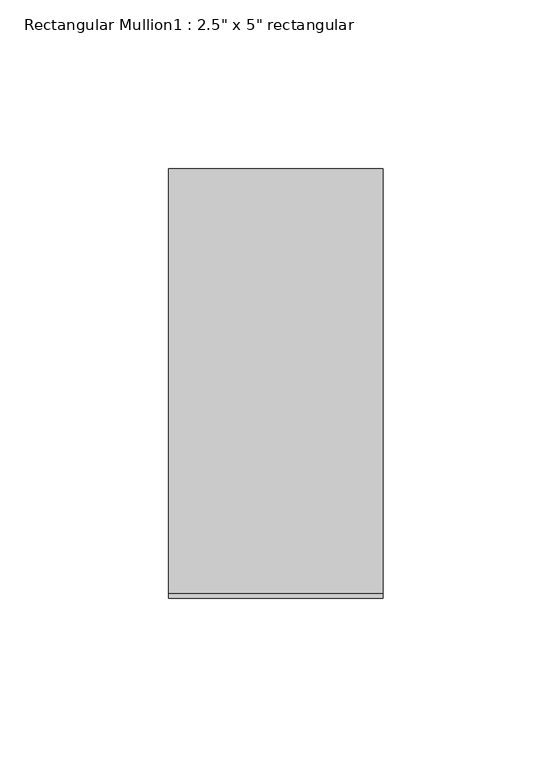
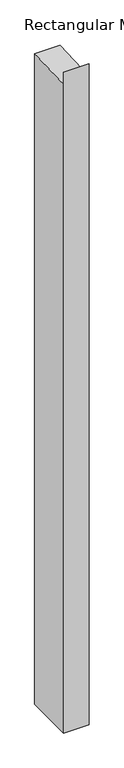
"""IFC4 building model written with IfcOpenShell, lengths in millimetres: member geometry."""

import ifcopenshell
import ifcopenshell.guid

model = None  # the IFC model being written
_history = None  # IfcOwnerHistory: only IFC2X3 demands one
_inside = {}  # id of a spatial element -> (the spatial element, [elements in it])
_under = {}  # id of a project, library or spatial element -> (it, [spatial elements below it])
_declared = {}  # id of a project -> (the project, [libraries it declares])
_typed = {}  # id of a type object -> (the type object, [elements of that type])
_made_of = {}  # id of a material, layer set ... -> (it, [elements and type objects made of it])


def new_model(schema):
    """Start an empty IFC model of exactly this schema.

    Asked for "IFC4X3", IfcOpenShell would pick the latest addendum, in which some entities
    have other attributes; the version numbers below select the first issue.
    IFC2X3 requires an IfcOwnerHistory on every rooted entity: one is made here for all.
    """
    global model, _history
    if schema == "IFC4X3":
        model = ifcopenshell.file(schema_version=(4, 3, 0, 0))
    else:
        model = ifcopenshell.file(schema=schema)
    _inside.clear()
    _under.clear()
    _declared.clear()
    _typed.clear()
    _made_of.clear()
    _history = None
    if model.schema == "IFC2X3":
        org = make("IfcOrganization", Name="unknown")
        user = make(
            "IfcPersonAndOrganization",
            ThePerson=make("IfcPerson", FamilyName="unknown"),
            TheOrganization=org,
        )
        app = make(
            "IfcApplication",
            ApplicationDeveloper=org,
            Version="unknown",
            ApplicationFullName="unknown",
            ApplicationIdentifier="unknown",
        )
        _history = make(
            "IfcOwnerHistory",
            OwningUser=user,
            OwningApplication=app,
            ChangeAction="ADDED",
            CreationDate=0,
        )
    return model


def make(cls, **values):
    """One entity of the class cls with the attributes given. An attribute that is None is left unset."""
    return model.create_entity(
        cls, **{name: value for name, value in values.items() if value is not None}
    )


def rooted(cls, **values):
    """An entity with a GlobalId (a new one), such as an element, a storey or a relation."""
    return make(cls, GlobalId=ifcopenshell.guid.new(), OwnerHistory=_history, **values)


def si_unit(unit_type, name, prefix=None):
    """IfcSIUnit, for example si_unit("LENGTHUNIT", "METRE", prefix="MILLI")."""
    return make("IfcSIUnit", UnitType=unit_type, Prefix=prefix, Name=name)


def assignment(units):
    """IfcUnitAssignment: the units of a project."""
    return None if units is None else make("IfcUnitAssignment", Units=units)


def point(xyz):
    """IfcCartesianPoint."""
    return None if xyz is None else make("IfcCartesianPoint", Coordinates=xyz)


def direction(xyz):
    """IfcDirection."""
    return None if xyz is None else make("IfcDirection", DirectionRatios=xyz)


def frame(location, z_axis=None, x_axis=None):
    """IfcAxis2Placement3D, a coordinate frame: its origin and axes. An axis left out is left unset."""
    return make(
        "IfcAxis2Placement3D",
        Location=point(location),
        Axis=direction(z_axis),
        RefDirection=direction(x_axis),
    )


def origin():
    """The frame at (0, 0, 0) with its axes left unset."""
    return frame((0.0, 0.0, 0.0))


def place(relative_to, where):
    """IfcLocalPlacement: puts the frame where relative to a parent placement (None: the world)."""
    return make(
        "IfcLocalPlacement", PlacementRelTo=relative_to, RelativePlacement=where
    )


def context(
    kind, dimensions, precision=None, world=None, true_north=None, identifier=None
):
    """IfcGeometricRepresentationContext, for example the 3D "Model" context."""
    return make(
        "IfcGeometricRepresentationContext",
        ContextIdentifier=identifier,
        ContextType=kind,
        CoordinateSpaceDimension=dimensions,
        Precision=precision,
        WorldCoordinateSystem=world,
        TrueNorth=true_north,
    )


def project(units=None, contexts=None):
    """IfcProject with its units and contexts."""
    return rooted(
        "IfcProject",
        Name="project",
        RepresentationContexts=contexts,
        UnitsInContext=assignment(units),
    )


def spatial(cls, under=None, at=None, **own):
    """A site, building, storey or space (cls), placed at a placement, below another one or the project."""
    s = rooted(cls, ObjectPlacement=at, **own)
    if under is not None:
        _under.setdefault(under.id(), (under, []))[1].append(s)
    return s


def polyline(points):
    """IfcPolyline through the points."""
    return make("IfcPolyline", Points=[point(p) for p in points])


def outline(outer, holes=None, kind="AREA"):
    """IfcArbitraryClosedProfileDef: a profile drawn as a closed curve; with holes, ...WithVoids."""
    if holes is None:
        return make("IfcArbitraryClosedProfileDef", ProfileType=kind, OuterCurve=outer)
    return make(
        "IfcArbitraryProfileDefWithVoids",
        ProfileType=kind,
        OuterCurve=outer,
        InnerCurves=holes,
    )


def extrude(swept, where, along, depth):
    """IfcExtrudedAreaSolid: the profile swept, set in the frame where, extruded along a direction by depth."""
    return make(
        "IfcExtrudedAreaSolid",
        SweptArea=swept,
        Position=where,
        ExtrudedDirection=direction(along),
        Depth=depth,
    )


def shape(context_of_items, identifier, shape_type, items):
    """IfcShapeRepresentation: the items that make up one representation, for example the "Body"."""
    return make(
        "IfcShapeRepresentation",
        ContextOfItems=context_of_items,
        RepresentationIdentifier=identifier,
        RepresentationType=shape_type,
        Items=items,
    )


def source(mapping_origin, context_of_items, identifier, shape_type, items):
    """IfcRepresentationMap: a shape defined once, which mapped items show again and again."""
    return make(
        "IfcRepresentationMap",
        MappingOrigin=mapping_origin,
        MappedRepresentation=shape(context_of_items, identifier, shape_type, items),
    )


def transform(
    local_origin,
    x_axis=None,
    y_axis=None,
    z_axis=None,
    scale=None,
    scale2=None,
    scale3=None,
    uniform=True,
):
    """IfcCartesianTransformationOperator3D, or its non-uniform kind. x_axis, y_axis, z_axis: its Axis1, 2, 3."""
    if uniform:
        return make(
            "IfcCartesianTransformationOperator3D",
            Axis1=direction(x_axis),
            Axis2=direction(y_axis),
            LocalOrigin=point(local_origin),
            Scale=scale,
            Axis3=direction(z_axis),
        )
    return make(
        "IfcCartesianTransformationOperator3DnonUniform",
        Axis1=direction(x_axis),
        Axis2=direction(y_axis),
        LocalOrigin=point(local_origin),
        Scale=scale,
        Axis3=direction(z_axis),
        Scale2=scale2,
        Scale3=scale3,
    )


def mapped(mapping_source, mapping_target):
    """IfcMappedItem: shows the shape of a source again, moved by a transform."""
    return make(
        "IfcMappedItem", MappingSource=mapping_source, MappingTarget=mapping_target
    )


def made_of(thing, what):
    """Note that an element or type object is made of a material, layer set ...; save() writes the relation."""
    if what is not None:
        _made_of.setdefault(what.id(), (what, []))[1].append(thing)
    return thing


def element(
    cls,
    number,
    at=None,
    inside=None,
    cuts=None,
    type_object=None,
    material=None,
    context=None,
    identifier="Body",
    shape_type=None,
    held_by="IfcProductDefinitionShape",
    body=None,
    shapes=None,
    **own,
):
    """One element of the class cls, such as IfcWall. Its Tag is "e" and its number.

    at: its placement. inside: the storey or other place that contains it. cuts: it is an
    opening in that element (IfcRelVoidsElement). A single representation is given by context,
    identifier, shape_type and body (its items); several are given by shapes. held_by: the class
    of the entity that holds the representations. save() writes the other relations.
    """
    e = rooted(cls, Tag="e%d" % number, ObjectPlacement=at, **own)
    if body is not None:
        shapes = [shape(context, identifier, shape_type, body)]
    if shapes is not None:
        e.Representation = make(held_by, Representations=shapes)
    if inside is not None:
        _inside.setdefault(inside.id(), (inside, []))[1].append(e)
    if cuts is not None:
        rooted(
            "IfcRelVoidsElement", RelatingBuildingElement=cuts, RelatedOpeningElement=e
        )
    if type_object is not None:
        _typed.setdefault(type_object.id(), (type_object, []))[1].append(e)
    return made_of(e, material)


def aggregate(whole, parts):
    """IfcRelAggregates: a whole, such as a stair, and the parts it consists of."""
    return rooted("IfcRelAggregates", RelatingObject=whole, RelatedObjects=parts)


def save(model, path):
    """Write the relations noted so far, then the file.

    IfcRelAggregates (storeys below a building ...), IfcRelContainedInSpatialStructure (elements
    in a storey), IfcRelDefinesByType, IfcRelAssociatesMaterial and IfcRelDeclares: one each for
    every whole, place, type object, material and project.
    """
    for whole, parts in _under.values():
        aggregate(whole, parts)
    for where, things in _inside.values():
        rooted(
            "IfcRelContainedInSpatialStructure",
            RelatedElements=things,
            RelatingStructure=where,
        )
    for kind, things in _typed.values():
        rooted("IfcRelDefinesByType", RelatedObjects=things, RelatingType=kind)
    for what, things in _made_of.values():
        rooted("IfcRelAssociatesMaterial", RelatedObjects=things, RelatingMaterial=what)
    for by, libraries in _declared.values():
        rooted("IfcRelDeclares", RelatingContext=by, RelatedDefinitions=libraries)
    model.write(path)


def member_0a0eb772(model_context):
    return source(origin(), model_context, "Body", "SweptSolid", [
        extrude(outline(polyline([(-63.5, 30.4748075), (-62.1741259, -2.5237591), (63.5, 2.5257955), (63.5, -1733.5500228), (-63.5, -1733.5500228), (-63.5, 30.4748075)])), frame((-63.5, 0.0, 0.0), z_axis=(1.0, 0.0, 0.0), x_axis=(0.0, 1.0, 0.0)), (0.0, 0.0, 1.0), 63.5),
    ])


if __name__ == "__main__":
    model = new_model("IFC4")
    model_context = context("Model", 3, world=origin())
    ifc_project = project(units=[si_unit("LENGTHUNIT", "METRE", prefix="MILLI")], contexts=[model_context])
    site = spatial("IfcSite", under=ifc_project)
    building = spatial("IfcBuilding", under=site)
    placement = place(None, origin())
    member_shape = member_0a0eb772(model_context)
    element("IfcMember", 1, ObjectType="Rectangular Mullion1 : 2.5\" x 5\" rectangular", at=placement, inside=building, context=model_context, shape_type="MappedRepresentation", body=[
        mapped(member_shape, transform((0.0, 0.0, 0.0), x_axis=(1.0, 0.0, 0.0), y_axis=(0.0, 1.0, 0.0), z_axis=(0.0, 0.0, 1.0))),
    ])
    save(model, "model.ifc")

# Revit data of these elements
# Type "Rectangular Mullion1 : 2.5\" x 5\" rectangular"
#   built-in parameter 1007304 = 0.416667 (stored number, unit not read)
#   built-in parameter 1007301 = 0.104167 (stored number, unit not read)
#   built-in parameter 1007300 = 0.104167 (stored number, unit not read)
# Element 1 (IfcMember, "Rectangular Mullion1 : 2.5\" x 5\" rectangular")
#   Materials on its faces: "support-frame"
# Materials
#   "support-frame": class "Unassigned", colour RGB 233 233 233, transparency 0, Cost = 0
